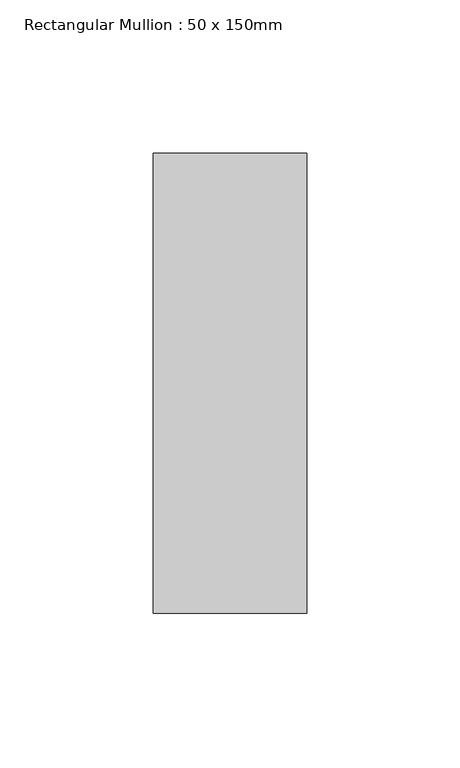
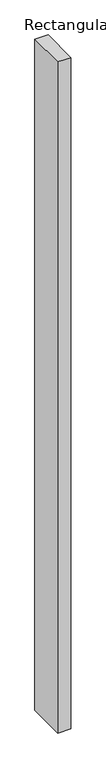
"""IFC4 building model written with IfcOpenShell, lengths in millimetres: member geometry, Rectangular Mullion : 50 x 150mm."""

from ifc_helpers import new_model, si_unit, frame, origin, place, context, project, spatial, polyline, outline, extrude, source, transform, mapped, element, save


def rectangular_mullion_50_x_150mm_929c4ac2(model_context):
    return source(origin(), model_context, "Body", "SweptSolid", [
        extrude(outline(polyline([(0.0, 75.0), (0.0, -75.0), (-50.0, -75.0), (-50.0, 75.0), (0.0, 75.0)])), frame((0.0, 0.0, -2700.0), z_axis=(0.0, 0.0, 1.0), x_axis=(1.0, 0.0, 0.0)), (0.0, 0.0, 1.0), 2700.0),
    ])


if __name__ == "__main__":
    model = new_model("IFC4")
    model_context = context("Model", 3, world=origin())
    ifc_project = project(units=[si_unit("LENGTHUNIT", "METRE", prefix="MILLI")], contexts=[model_context])
    site = spatial("IfcSite", under=ifc_project)
    building = spatial("IfcBuilding", under=site)
    placement = place(None, origin())
    rectangular_mullion_50_x_150mm_shape = rectangular_mullion_50_x_150mm_929c4ac2(model_context)
    element("IfcMember", 1, ObjectType="Rectangular Mullion : 50 x 150mm", at=placement, inside=building, context=model_context, shape_type="MappedRepresentation", body=[
        mapped(rectangular_mullion_50_x_150mm_shape, transform((0.0, 0.0, 0.0), x_axis=(1.0, 0.0, 0.0), y_axis=(0.0, 1.0, 0.0), z_axis=(0.0, 0.0, 1.0))),
    ])
    save(model, "model.ifc")

# Revit data of these elements
# Type "Rectangular Mullion : 50 x 150mm"
#   built-in parameter 1007304 = 0.492126 (stored number, unit not read)
#   built-in parameter 1007301 = 0.082021 (stored number, unit not read)
#   built-in parameter 1007300 = 0.082021 (stored number, unit not read)
# Element 1 (IfcMember, "Rectangular Mullion : 50 x 150mm")
#   Materials on its faces: "Metal - Aluminium"
# Materials
#   "Metal - Aluminium": class "Metal", colour RGB 247 247 247, transparency 0
